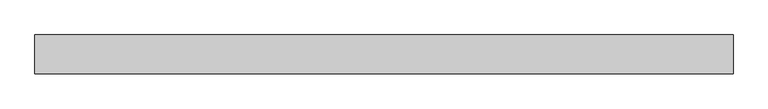
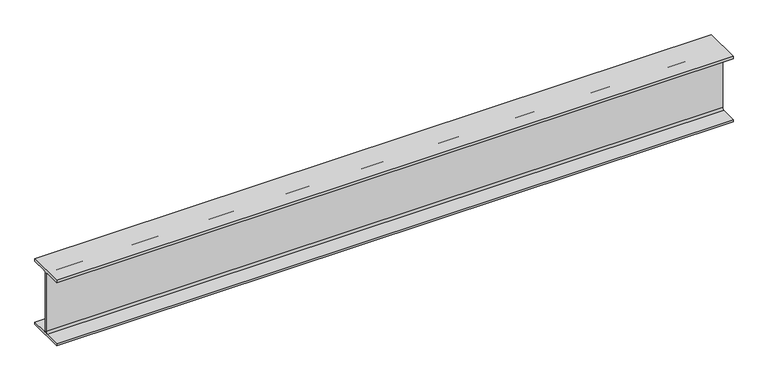
"""IFC4 building model written with IfcOpenShell, lengths in millimetres: beam geometry, Old_Steel Beam_H-KSD3502 : H_SB_ASB_H-200×200x8x12."""

from ifc_helpers import new_model, si_unit, point, frame, frame_2d, origin, place, context, project, spatial, polyline, circle_curve, trimmed, segment, composite_curve, outline, extrude, source, transform, mapped, element, save


def beam_97ed9082(model_context):
    return source(origin(), model_context, "Body", "SweptSolid", [
        extrude(outline(composite_curve([segment(polyline([(82.5, -141.5), (82.5, -151.7), (-82.5, -151.7), (-82.5, -141.5), (-11.9, -141.5)]), True, "CONTINUOUS"), segment(trimmed(circle_curve(frame_2d((-11.9, -132.6)), 8.9), [point((-11.9, -141.5))], [point((-3.0, -132.6))], True, "CARTESIAN"), True, "CONTINUOUS"), segment(polyline([(-3.0, -132.6), (-3.0, 132.6)]), True, "CONTINUOUS"), segment(trimmed(circle_curve(frame_2d((-11.9, 132.6)), 8.9), [point((-3.0, 132.6))], [point((-11.9, 141.5))], True, "CARTESIAN"), True, "CONTINUOUS"), segment(polyline([(-11.9, 141.5), (-82.5, 141.5), (-82.5, 151.7), (82.5, 151.7), (82.5, 141.5), (11.9, 141.5)]), True, "CONTINUOUS"), segment(trimmed(circle_curve(frame_2d((11.9, 132.6)), 8.9), [point((11.9, 141.5))], [point((3.0, 132.6))], True, "CARTESIAN"), True, "CONTINUOUS"), segment(polyline([(3.0, 132.6), (3.0, -132.6)]), True, "CONTINUOUS"), segment(trimmed(circle_curve(frame_2d((11.9, -132.6)), 8.9), [point((3.0, -132.6))], [point((11.9, -141.5))], True, "CARTESIAN"), True, "CONTINUOUS"), segment(polyline([(11.9, -141.5), (82.5, -141.5)]), True, "CONTINUOUS")], self_intersect=False)), frame((-1443.5851857, 0.0, 0.0), z_axis=(1.0, 0.0, 0.0), x_axis=(0.0, 1.0, 0.0)), (0.0, 0.0, 1.0), 2972.6935261),
    ])


if __name__ == "__main__":
    model = new_model("IFC4")
    model_context = context("Model", 3, world=origin())
    ifc_project = project(units=[si_unit("LENGTHUNIT", "METRE", prefix="MILLI")], contexts=[model_context])
    site = spatial("IfcSite", under=ifc_project)
    building = spatial("IfcBuilding", under=site)
    placement = place(None, origin())
    beam_shape = beam_97ed9082(model_context)
    element("IfcBeam", 1, ObjectType="Old_Steel Beam_H-KSD3502 : H_SB_ASB_H-200×200x8x12", at=placement, inside=building, context=model_context, shape_type="MappedRepresentation", body=[
        mapped(beam_shape, transform((0.0, 0.0, 0.0), x_axis=(1.0, 0.0, 0.0), y_axis=(0.0, 1.0, 0.0), z_axis=(0.0, 0.0, 1.0))),
    ])
    save(model, "model.ifc")

# Revit data of these elements
# Type "Old_Steel Beam_H-KSD3502 : H_SB_ASB_H-200×200x8x12"
#   Width = 20.0 cm
#   Web Thickness = 0.8 cm
#   Web Fillet = 1.3 cm
#   Warping Constant = 141376.0 cm⁶
#   Torsional Moment of Inertia = 26.2485 cm⁴
#   Torsional Modulus = 1.0 cm³
#   Section Area = 63.53 cm²
#   Plastic Modulus weak axis = 244.0 cm³
#   Plastic Modulus strong axis = 525.0 cm³
#   Perimeter = 1.16 m²/m
#   Nominal Weight = 49.90 kgf/m
#   Moment of Inertia weak axis = 1600.00 cm⁴
#   Moment of Inertia strong axis = 4720.00 cm⁴
#   Height = 20.0 cm
#   Flange Thickness = 1.2 cm
#   Elastic Modulus weak axis = 160.0 cm³
#   Elastic Modulus strong axis = 472.0 cm³
#   Centroid Vertical = 10.0 cm
#   Centroid Horizontal = 10.0 cm
#   Length [instance default] = 1.5240 m
#   Structural Material [instance default] = Steel, 45-345
#   Assembly Code = ""
# Element 1 (IfcBeam, "Old_Steel Beam_H-KSD3502 : H_SB_ASB_H-200×200x8x12")
#   Structural Material = none
# Materials
#   "Steel, 45-345": class "Metal", colour RGB 189 187 185, transparency 0, Description = "Steel 345 MPa", Cost = 0
